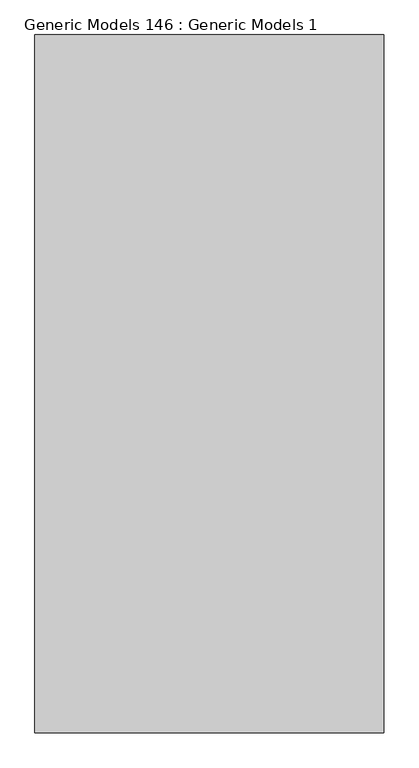
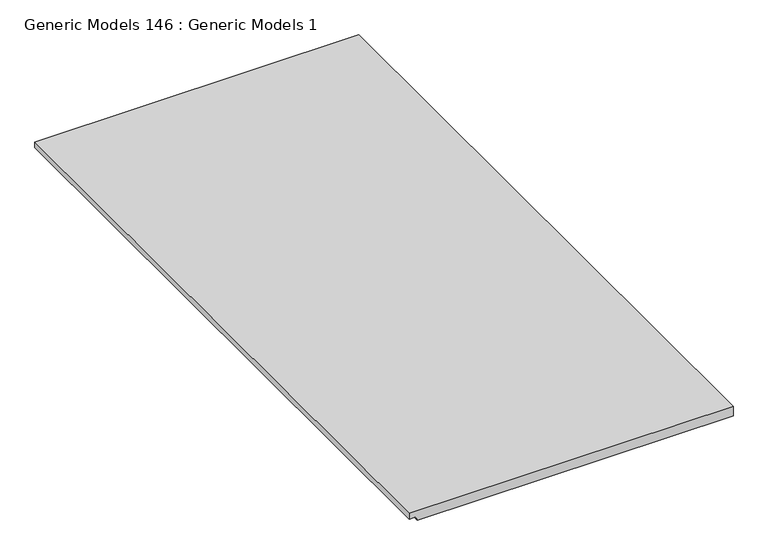
"""IFC4 building model written with IfcOpenShell, lengths in millimetres: proxy geometry, Generic Models 146 : Generic Models 1."""

from ifc_helpers import new_model, si_unit, frame, origin, place, context, project, spatial, polyline, outline, extrude, source, transform, mapped, element, save


def generic_models_146_generic_models_1_64768bb5(model_context):
    return source(origin(), model_context, "Body", "SweptSolid", [
        extrude(outline(polyline([(2027.354361, 46965.2186938), (2016.241861, 46965.2186938), (2016.241861, 46977.9186938), (2008.304361, 46980.8077075), (2008.304361, 47574.8186938), (2027.354361, 47574.8186938), (2027.354361, 46965.2186938)])), frame((0.0, 0.0, 0.0), z_axis=(0.0, 1.0, 0.0), x_axis=(0.0, 0.0, 1.0)), (0.0, 0.0, 1.0), 1219.2),
    ])


if __name__ == "__main__":
    model = new_model("IFC4")
    model_context = context("Model", 3, world=origin())
    ifc_project = project(units=[si_unit("LENGTHUNIT", "METRE", prefix="MILLI")], contexts=[model_context])
    site = spatial("IfcSite", under=ifc_project)
    building = spatial("IfcBuilding", under=site)
    placement = place(None, origin())
    generic_models_146_generic_models_1_shape = generic_models_146_generic_models_1_64768bb5(model_context)
    element("IfcBuildingElementProxy", 1, Name="Generic Models 146 : Generic Models 1", ObjectType="Generic Models 146 : Generic Models 1", at=placement, inside=building, context=model_context, shape_type="MappedRepresentation", body=[
        mapped(generic_models_146_generic_models_1_shape, transform((0.0, 0.0, 0.0), x_axis=(1.0, 0.0, 0.0), y_axis=(0.0, 1.0, 0.0), z_axis=(0.0, 0.0, 1.0))),
    ])
    save(model, "model.ifc")

# Revit data of these elements
# Element 1 (IfcBuildingElementProxy, "Generic Models 146 : Generic Models 1")
#   Materials on its faces: "CEILING AS SCHEDULED"
# Materials
#   "CEILING AS SCHEDULED": class "Generic", colour RGB 255 255 255, transparency 0, Cost = 0
